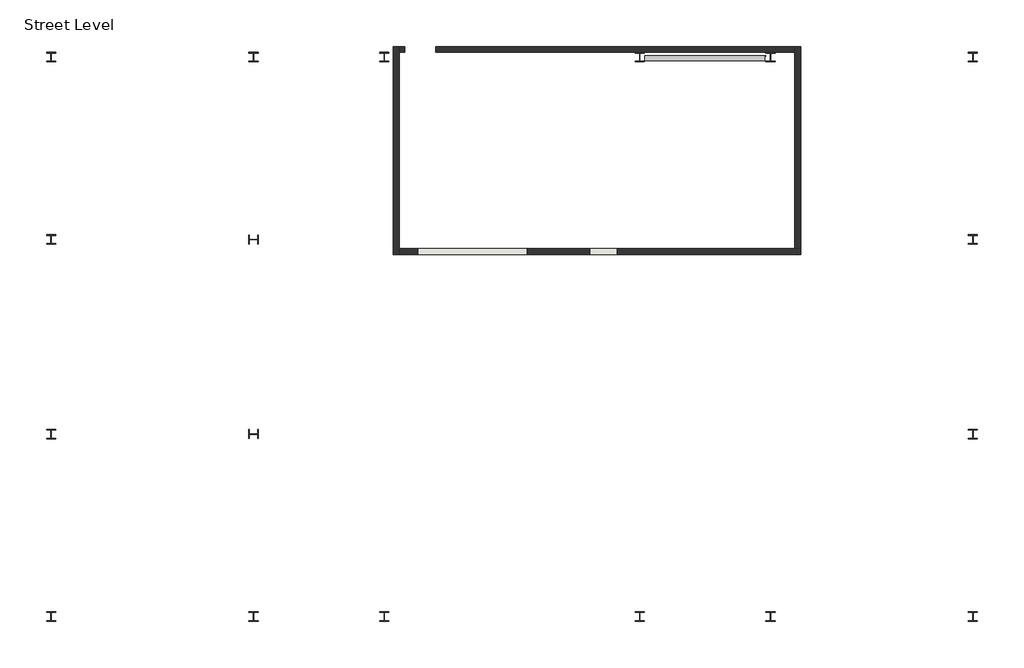
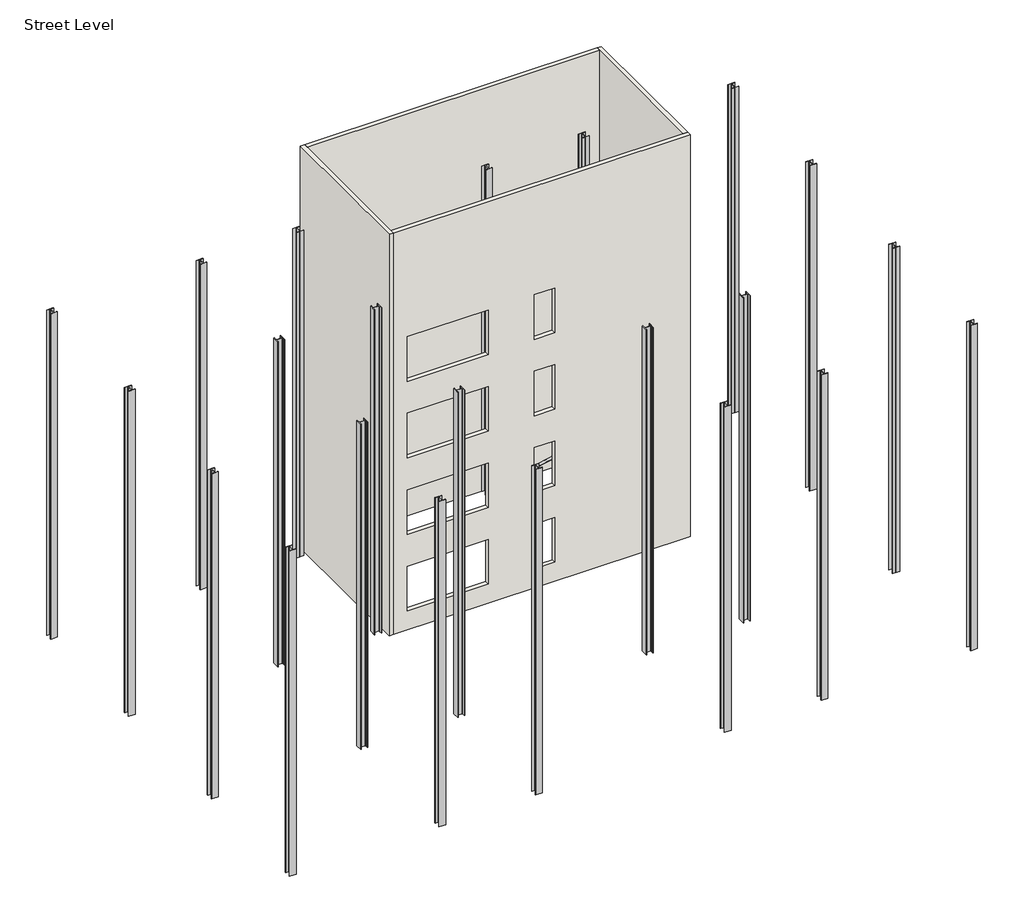
# One storey: 24 columns, 4 walls, 1 member.
"""IFC4 building model written with IfcOpenShell, lengths in millimetres."""

import ifcopenshell
import ifcopenshell.guid

model = None  # the IFC model being written
_history = None  # IfcOwnerHistory: only IFC2X3 demands one
_inside = {}  # id of a spatial element -> (the spatial element, [elements in it])
_under = {}  # id of a project, library or spatial element -> (it, [spatial elements below it])
_declared = {}  # id of a project -> (the project, [libraries it declares])
_typed = {}  # id of a type object -> (the type object, [elements of that type])
_made_of = {}  # id of a material, layer set ... -> (it, [elements and type objects made of it])


def new_model(schema):
    """Start an empty IFC model of exactly this schema.

    Asked for "IFC4X3", IfcOpenShell would pick the latest addendum, in which some entities
    have other attributes; the version numbers below select the first issue.
    IFC2X3 requires an IfcOwnerHistory on every rooted entity: one is made here for all.
    """
    global model, _history
    if schema == "IFC4X3":
        model = ifcopenshell.file(schema_version=(4, 3, 0, 0))
    else:
        model = ifcopenshell.file(schema=schema)
    _inside.clear()
    _under.clear()
    _declared.clear()
    _typed.clear()
    _made_of.clear()
    _history = None
    if model.schema == "IFC2X3":
        org = make("IfcOrganization", Name="unknown")
        user = make(
            "IfcPersonAndOrganization",
            ThePerson=make("IfcPerson", FamilyName="unknown"),
            TheOrganization=org,
        )
        app = make(
            "IfcApplication",
            ApplicationDeveloper=org,
            Version="unknown",
            ApplicationFullName="unknown",
            ApplicationIdentifier="unknown",
        )
        _history = make(
            "IfcOwnerHistory",
            OwningUser=user,
            OwningApplication=app,
            ChangeAction="ADDED",
            CreationDate=0,
        )
    return model


def make(cls, **values):
    """One entity of the class cls with the attributes given. An attribute that is None is left unset."""
    return model.create_entity(
        cls, **{name: value for name, value in values.items() if value is not None}
    )


def rooted(cls, **values):
    """An entity with a GlobalId (a new one), such as an element, a storey or a relation."""
    return make(cls, GlobalId=ifcopenshell.guid.new(), OwnerHistory=_history, **values)


def si_unit(unit_type, name, prefix=None):
    """IfcSIUnit, for example si_unit("LENGTHUNIT", "METRE", prefix="MILLI")."""
    return make("IfcSIUnit", UnitType=unit_type, Prefix=prefix, Name=name)


def assignment(units):
    """IfcUnitAssignment: the units of a project."""
    return None if units is None else make("IfcUnitAssignment", Units=units)


def point(xyz):
    """IfcCartesianPoint."""
    return None if xyz is None else make("IfcCartesianPoint", Coordinates=xyz)


def direction(xyz):
    """IfcDirection."""
    return None if xyz is None else make("IfcDirection", DirectionRatios=xyz)


def frame(location, z_axis=None, x_axis=None):
    """IfcAxis2Placement3D, a coordinate frame: its origin and axes. An axis left out is left unset."""
    return make(
        "IfcAxis2Placement3D",
        Location=point(location),
        Axis=direction(z_axis),
        RefDirection=direction(x_axis),
    )


def frame_2d(location, x_axis=None):
    """IfcAxis2Placement2D, a coordinate frame in the plane: its origin and x axis."""
    return make(
        "IfcAxis2Placement2D", Location=point(location), RefDirection=direction(x_axis)
    )


def origin():
    """The frame at (0, 0, 0) with its axes left unset."""
    return frame((0.0, 0.0, 0.0))


def place(relative_to, where):
    """IfcLocalPlacement: puts the frame where relative to a parent placement (None: the world)."""
    return make(
        "IfcLocalPlacement", PlacementRelTo=relative_to, RelativePlacement=where
    )


def context(
    kind, dimensions, precision=None, world=None, true_north=None, identifier=None
):
    """IfcGeometricRepresentationContext, for example the 3D "Model" context."""
    return make(
        "IfcGeometricRepresentationContext",
        ContextIdentifier=identifier,
        ContextType=kind,
        CoordinateSpaceDimension=dimensions,
        Precision=precision,
        WorldCoordinateSystem=world,
        TrueNorth=true_north,
    )


def project(units=None, contexts=None):
    """IfcProject with its units and contexts."""
    return rooted(
        "IfcProject",
        Name="project",
        RepresentationContexts=contexts,
        UnitsInContext=assignment(units),
    )


def spatial(cls, under=None, at=None, **own):
    """A site, building, storey or space (cls), placed at a placement, below another one or the project."""
    s = rooted(cls, ObjectPlacement=at, **own)
    if under is not None:
        _under.setdefault(under.id(), (under, []))[1].append(s)
    return s


def polyline(points):
    """IfcPolyline through the points."""
    return make("IfcPolyline", Points=[point(p) for p in points])


def circle_curve(where, radius):
    """IfcCircle in the frame where."""
    return make("IfcCircle", Position=where, Radius=radius)


def trimmed(basis, trim1, trim2, sense, master):
    """IfcTrimmedCurve: the piece of a basis curve between two trims."""
    return make(
        "IfcTrimmedCurve",
        BasisCurve=basis,
        Trim1=trim1,
        Trim2=trim2,
        SenseAgreement=sense,
        MasterRepresentation=master,
    )


def segment(curve, same_sense, transition):
    """IfcCompositeCurveSegment."""
    return make(
        "IfcCompositeCurveSegment",
        Transition=transition,
        SameSense=same_sense,
        ParentCurve=curve,
    )


def composite_curve(segments, self_intersect=None):
    """IfcCompositeCurve: segments joined end to end."""
    return make("IfcCompositeCurve", Segments=segments, SelfIntersect=self_intersect)


def outline(outer, holes=None, kind="AREA"):
    """IfcArbitraryClosedProfileDef: a profile drawn as a closed curve; with holes, ...WithVoids."""
    if holes is None:
        return make("IfcArbitraryClosedProfileDef", ProfileType=kind, OuterCurve=outer)
    return make(
        "IfcArbitraryProfileDefWithVoids",
        ProfileType=kind,
        OuterCurve=outer,
        InnerCurves=holes,
    )


def extrude(swept, where, along, depth):
    """IfcExtrudedAreaSolid: the profile swept, set in the frame where, extruded along a direction by depth."""
    return make(
        "IfcExtrudedAreaSolid",
        SweptArea=swept,
        Position=where,
        ExtrudedDirection=direction(along),
        Depth=depth,
    )


def faces_of(points, faces, orient=None, outer=None):
    """IfcFace entities. A face is a list of loops; a loop is a list of indices into points, from 0.

    orient and outer hold one flag for each loop. By default every Orientation is true, the
    first loop of a face is its IfcFaceOuterBound and the others are IfcFaceBound.
    """
    made = []
    for i, loops in enumerate(faces):
        bounds = []
        for j, loop in enumerate(loops):
            is_outer = j == 0 if outer is None else outer[i][j]
            bounds.append(
                make(
                    "IfcFaceOuterBound" if is_outer else "IfcFaceBound",
                    Bound=make("IfcPolyLoop", Polygon=[points[k] for k in loop]),
                    Orientation=True if orient is None else orient[i][j],
                )
            )
        made.append(make("IfcFace", Bounds=bounds))
    return made


def faceted_brep(points, faces, orient=None, outer=None, voids=None):
    """IfcFacetedBrep: a solid bounded by flat faces; with voids (closed shells), ...WithVoids."""
    shared = [point(p) for p in points]
    hull = make("IfcClosedShell", CfsFaces=faces_of(shared, faces, orient, outer))
    if voids is None:
        return make("IfcFacetedBrep", Outer=hull)
    return make(
        "IfcFacetedBrepWithVoids",
        Outer=hull,
        Voids=[
            make(cls, CfsFaces=faces_of(shared, fs, o, b)) for cls, fs, o, b in voids
        ],
    )


def shape(context_of_items, identifier, shape_type, items):
    """IfcShapeRepresentation: the items that make up one representation, for example the "Body"."""
    return make(
        "IfcShapeRepresentation",
        ContextOfItems=context_of_items,
        RepresentationIdentifier=identifier,
        RepresentationType=shape_type,
        Items=items,
    )


def source(mapping_origin, context_of_items, identifier, shape_type, items):
    """IfcRepresentationMap: a shape defined once, which mapped items show again and again."""
    return make(
        "IfcRepresentationMap",
        MappingOrigin=mapping_origin,
        MappedRepresentation=shape(context_of_items, identifier, shape_type, items),
    )


def transform(
    local_origin,
    x_axis=None,
    y_axis=None,
    z_axis=None,
    scale=None,
    scale2=None,
    scale3=None,
    uniform=True,
):
    """IfcCartesianTransformationOperator3D, or its non-uniform kind. x_axis, y_axis, z_axis: its Axis1, 2, 3."""
    if uniform:
        return make(
            "IfcCartesianTransformationOperator3D",
            Axis1=direction(x_axis),
            Axis2=direction(y_axis),
            LocalOrigin=point(local_origin),
            Scale=scale,
            Axis3=direction(z_axis),
        )
    return make(
        "IfcCartesianTransformationOperator3DnonUniform",
        Axis1=direction(x_axis),
        Axis2=direction(y_axis),
        LocalOrigin=point(local_origin),
        Scale=scale,
        Axis3=direction(z_axis),
        Scale2=scale2,
        Scale3=scale3,
    )


def mapped(mapping_source, mapping_target):
    """IfcMappedItem: shows the shape of a source again, moved by a transform."""
    return make(
        "IfcMappedItem", MappingSource=mapping_source, MappingTarget=mapping_target
    )


def made_of(thing, what):
    """Note that an element or type object is made of a material, layer set ...; save() writes the relation."""
    if what is not None:
        _made_of.setdefault(what.id(), (what, []))[1].append(thing)
    return thing


def element(
    cls,
    number,
    at=None,
    inside=None,
    cuts=None,
    type_object=None,
    material=None,
    context=None,
    identifier="Body",
    shape_type=None,
    held_by="IfcProductDefinitionShape",
    body=None,
    shapes=None,
    **own,
):
    """One element of the class cls, such as IfcWall. Its Tag is "e" and its number.

    at: its placement. inside: the storey or other place that contains it. cuts: it is an
    opening in that element (IfcRelVoidsElement). A single representation is given by context,
    identifier, shape_type and body (its items); several are given by shapes. held_by: the class
    of the entity that holds the representations. save() writes the other relations.
    """
    e = rooted(cls, Tag="e%d" % number, ObjectPlacement=at, **own)
    if body is not None:
        shapes = [shape(context, identifier, shape_type, body)]
    if shapes is not None:
        e.Representation = make(held_by, Representations=shapes)
    if inside is not None:
        _inside.setdefault(inside.id(), (inside, []))[1].append(e)
    if cuts is not None:
        rooted(
            "IfcRelVoidsElement", RelatingBuildingElement=cuts, RelatedOpeningElement=e
        )
    if type_object is not None:
        _typed.setdefault(type_object.id(), (type_object, []))[1].append(e)
    return made_of(e, material)


def aggregate(whole, parts):
    """IfcRelAggregates: a whole, such as a stair, and the parts it consists of."""
    return rooted("IfcRelAggregates", RelatingObject=whole, RelatedObjects=parts)


def save(model, path):
    """Write the relations noted so far, then the file.

    IfcRelAggregates (storeys below a building ...), IfcRelContainedInSpatialStructure (elements
    in a storey), IfcRelDefinesByType, IfcRelAssociatesMaterial and IfcRelDeclares: one each for
    every whole, place, type object, material and project.
    """
    for whole, parts in _under.values():
        aggregate(whole, parts)
    for where, things in _inside.values():
        rooted(
            "IfcRelContainedInSpatialStructure",
            RelatedElements=things,
            RelatingStructure=where,
        )
    for kind, things in _typed.values():
        rooted("IfcRelDefinesByType", RelatedObjects=things, RelatingType=kind)
    for what, things in _made_of.values():
        rooted("IfcRelAssociatesMaterial", RelatedObjects=things, RelatingMaterial=what)
    for by, libraries in _declared.values():
        rooted("IfcRelDeclares", RelatingContext=by, RelatedDefinitions=libraries)
    model.write(path)


def w_wide_flange_column_w12x87_da20b1fb(model_context):
    return source(origin(), model_context, "Body", "SweptSolid", [
        extrude(outline(composite_curve([segment(polyline([(153.9875, 159.146875), (153.9875, 138.6085937), (28.8726562, 138.6085937)]), True, "CONTINUOUS"), segment(trimmed(circle_curve(frame_2d((28.8726562, 116.284375)), 22.3242188), [point((28.8726562, 138.6085937))], [point((6.5484375, 116.284375))], True, "CARTESIAN"), True, "CONTINUOUS"), segment(polyline([(6.5484375, 116.284375), (6.5484375, -116.284375)]), True, "CONTINUOUS"), segment(trimmed(circle_curve(frame_2d((28.8726562, -116.284375)), 22.3242188), [point((6.5484375, -116.284375))], [point((28.8726562, -138.6085937))], True, "CARTESIAN"), True, "CONTINUOUS"), segment(polyline([(28.8726562, -138.6085937), (153.9875, -138.6085937), (153.9875, -159.146875), (-153.9875, -159.146875), (-153.9875, -138.6085937), (-28.8726563, -138.6085937)]), True, "CONTINUOUS"), segment(trimmed(circle_curve(frame_2d((-28.8726563, -116.284375)), 22.3242188), [point((-28.8726563, -138.6085937))], [point((-6.5484375, -116.284375))], True, "CARTESIAN"), True, "CONTINUOUS"), segment(polyline([(-6.5484375, -116.284375), (-6.5484375, 116.284375)]), True, "CONTINUOUS"), segment(trimmed(circle_curve(frame_2d((-28.8726563, 116.284375)), 22.3242188), [point((-6.5484375, 116.284375))], [point((-28.8726563, 138.6085937))], True, "CARTESIAN"), True, "CONTINUOUS"), segment(polyline([(-28.8726563, 138.6085937), (-153.9875, 138.6085937), (-153.9875, 159.146875), (153.9875, 159.146875)]), True, "CONTINUOUS")], self_intersect=False)), frame((0.0, 0.0, -914.4), z_axis=(0.0, 0.0, 1.0), x_axis=(1.0, 0.0, 0.0)), (0.0, 0.0, 1.0), 15544.8),
    ])


def l_angle2_l6x6x3_8_670392f0(model_context):
    return source(origin(), model_context, "Body", "SweptSolid", [
        extrude(outline(composite_curve([segment(polyline([(41.148, 41.148), (41.148, -111.252)]), True, "CONTINUOUS"), segment(trimmed(circle_curve(frame_2d((41.148, -101.727)), 9.525), [point((41.148, -111.252))], [point((31.623, -101.727))], False, "CARTESIAN"), True, "CONTINUOUS"), segment(polyline([(31.623, -101.727), (31.623, 22.098)]), True, "CONTINUOUS"), segment(trimmed(circle_curve(frame_2d((22.098, 22.098)), 9.525), [point((31.623, 22.098))], [point((22.098, 31.623))], True, "CARTESIAN"), True, "CONTINUOUS"), segment(polyline([(22.098, 31.623), (-101.727, 31.623)]), True, "CONTINUOUS"), segment(trimmed(circle_curve(frame_2d((-101.727, 41.148)), 9.525), [point((-101.727, 31.623))], [point((-111.252, 41.148))], False, "CARTESIAN"), True, "CONTINUOUS"), segment(polyline([(-111.252, 41.148), (41.148, 41.148)]), True, "CONTINUOUS")], self_intersect=False)), frame((-2053.0970548, 0.0, 0.0), z_axis=(1.0, 0.0, 0.0), x_axis=(0.0, 1.0, 0.0)), (0.0, 0.0, 1.0), 4091.5211794),
    ])


model = new_model("IFC4")

# Units and contexts
model_context = context("Model", 3, world=origin())
ifc_project = project(units=[si_unit("LENGTHUNIT", "METRE", prefix="MILLI")], contexts=[model_context])

# Site, building, storey
site = spatial("IfcSite", under=ifc_project)
building = spatial("IfcBuilding", under=site)
storey = spatial("IfcBuildingStorey", under=building, Name="Street Level", Elevation=-914.4)

# Columns
placement = place(None, origin())
w_wide_flange_column_w12x87_shape = w_wide_flange_column_w12x87_da20b1fb(model_context)
element("IfcColumn", 1, ObjectType="W-Wide Flange-Column : W12X87", at=placement, inside=storey, context=model_context, shape_type="MappedRepresentation", body=[
    mapped(w_wide_flange_column_w12x87_shape, transform((-9801.8122732, -3408.4984696, 0.0), x_axis=(0.0, -1.0, 0.0), y_axis=(1.0, 0.0, 0.0), z_axis=(0.0, 0.0, 1.0))),
])
element("IfcColumn", 2, ObjectType="W-Wide Flange-Column : W12X87", at=placement, inside=storey, context=model_context, shape_type="MappedRepresentation", body=[
    mapped(w_wide_flange_column_w12x87_shape, transform((-5433.0122732, -3408.4984696, 0.0), x_axis=(0.0, -1.0, 0.0), y_axis=(1.0, 0.0, 0.0), z_axis=(0.0, 0.0, 1.0))),
])
element("IfcColumn", 3, ObjectType="W-Wide Flange-Column : W12X87", at=placement, inside=storey, context=model_context, shape_type="MappedRepresentation", body=[
    mapped(w_wide_flange_column_w12x87_shape, transform((3101.3877268, -3408.4984696, 0.0), x_axis=(0.0, -1.0, 0.0), y_axis=(1.0, 0.0, 0.0), z_axis=(0.0, 0.0, 1.0))),
])
element("IfcColumn", 4, ObjectType="W-Wide Flange-Column : W12X87", at=placement, inside=storey, context=model_context, shape_type="MappedRepresentation", body=[
    mapped(w_wide_flange_column_w12x87_shape, transform((7470.1877268, -3408.4984696, 0.0), x_axis=(0.0, -1.0, 0.0), y_axis=(1.0, 0.0, 0.0), z_axis=(0.0, 0.0, 1.0))),
])
element("IfcColumn", 5, ObjectType="W-Wide Flange-Column : W12X87", at=placement, inside=storey, context=model_context, shape_type="MappedRepresentation", body=[
    mapped(w_wide_flange_column_w12x87_shape, transform((-9801.8122732, 3093.9015304, 0.0), x_axis=(0.0, -1.0, 0.0), y_axis=(1.0, 0.0, 0.0), z_axis=(0.0, 0.0, 1.0))),
])
element("IfcColumn", 6, ObjectType="W-Wide Flange-Column : W12X87", at=placement, inside=storey, context=model_context, shape_type="MappedRepresentation", body=[
    mapped(w_wide_flange_column_w12x87_shape, transform((-5433.0122732, 3093.9015304, 0.0), x_axis=(0.0, -1.0, 0.0), y_axis=(1.0, 0.0, 0.0), z_axis=(0.0, 0.0, 1.0))),
])
element("IfcColumn", 7, ObjectType="W-Wide Flange-Column : W12X87", at=placement, inside=storey, context=model_context, shape_type="MappedRepresentation", body=[
    mapped(w_wide_flange_column_w12x87_shape, transform((3101.3877268, 3093.9015304, 0.0), x_axis=(0.0, -1.0, 0.0), y_axis=(1.0, 0.0, 0.0), z_axis=(0.0, 0.0, 1.0))),
])
element("IfcColumn", 8, ObjectType="W-Wide Flange-Column : W12X87", at=placement, inside=storey, context=model_context, shape_type="MappedRepresentation", body=[
    mapped(w_wide_flange_column_w12x87_shape, transform((7470.1877268, 3093.9015304, 0.0), x_axis=(0.0, -1.0, 0.0), y_axis=(1.0, 0.0, 0.0), z_axis=(0.0, 0.0, 1.0))),
])
element("IfcColumn", 9, ObjectType="W-Wide Flange-Column : W12X87", at=placement, inside=storey, context=model_context, shape_type="MappedRepresentation", body=[
    mapped(w_wide_flange_column_w12x87_shape, transform((-16558.2122732, 9189.9015304, 0.0), x_axis=(1.0, 0.0, 0.0), y_axis=(0.0, 1.0, 0.0), z_axis=(0.0, 0.0, 1.0))),
])
element("IfcColumn", 10, ObjectType="W-Wide Flange-Column : W12X87", at=placement, inside=storey, context=model_context, shape_type="MappedRepresentation", body=[
    mapped(w_wide_flange_column_w12x87_shape, transform((-16558.2122732, 3093.9015304, 0.0), x_axis=(1.0, 0.0, 0.0), y_axis=(0.0, 1.0, 0.0), z_axis=(0.0, 0.0, 1.0))),
])
element("IfcColumn", 11, ObjectType="W-Wide Flange-Column : W12X87", at=placement, inside=storey, context=model_context, shape_type="MappedRepresentation", body=[
    mapped(w_wide_flange_column_w12x87_shape, transform((-9801.8122732, 9189.9015304, 0.0), x_axis=(1.0, 0.0, 0.0), y_axis=(0.0, 1.0, 0.0), z_axis=(0.0, 0.0, 1.0))),
])
element("IfcColumn", 12, ObjectType="W-Wide Flange-Column : W12X87", at=placement, inside=storey, context=model_context, shape_type="MappedRepresentation", body=[
    mapped(w_wide_flange_column_w12x87_shape, transform((-5433.0122732, 9189.9015304, 0.0), x_axis=(1.0, 0.0, 0.0), y_axis=(0.0, 1.0, 0.0), z_axis=(0.0, 0.0, 1.0))),
])
element("IfcColumn", 13, ObjectType="W-Wide Flange-Column : W12X87", at=placement, inside=storey, context=model_context, shape_type="MappedRepresentation", body=[
    mapped(w_wide_flange_column_w12x87_shape, transform((3101.3877268, 9189.9015304, 0.0), x_axis=(1.0, 0.0, 0.0), y_axis=(0.0, 1.0, 0.0), z_axis=(0.0, 0.0, 1.0))),
])
element("IfcColumn", 14, ObjectType="W-Wide Flange-Column : W12X87", at=placement, inside=storey, context=model_context, shape_type="MappedRepresentation", body=[
    mapped(w_wide_flange_column_w12x87_shape, transform((7470.1877268, 9189.9015304, 0.0), x_axis=(1.0, 0.0, 0.0), y_axis=(0.0, 1.0, 0.0), z_axis=(0.0, 0.0, 1.0))),
])
element("IfcColumn", 15, ObjectType="W-Wide Flange-Column : W12X87", at=placement, inside=storey, context=model_context, shape_type="MappedRepresentation", body=[
    mapped(w_wide_flange_column_w12x87_shape, transform((14226.5877268, 9189.9015304, 0.0), x_axis=(1.0, 0.0, 0.0), y_axis=(0.0, 1.0, 0.0), z_axis=(0.0, 0.0, 1.0))),
])
element("IfcColumn", 16, ObjectType="W-Wide Flange-Column : W12X87", at=placement, inside=storey, context=model_context, shape_type="MappedRepresentation", body=[
    mapped(w_wide_flange_column_w12x87_shape, transform((14226.5877268, 3093.9015304, 0.0), x_axis=(1.0, 0.0, 0.0), y_axis=(0.0, 1.0, 0.0), z_axis=(0.0, 0.0, 1.0))),
])
element("IfcColumn", 17, ObjectType="W-Wide Flange-Column : W12X87", at=placement, inside=storey, context=model_context, shape_type="MappedRepresentation", body=[
    mapped(w_wide_flange_column_w12x87_shape, transform((14226.5877268, -3408.4984696, 0.0), x_axis=(1.0, 0.0, 0.0), y_axis=(0.0, 1.0, 0.0), z_axis=(0.0, 0.0, 1.0))),
])
element("IfcColumn", 18, ObjectType="W-Wide Flange-Column : W12X87", at=placement, inside=storey, context=model_context, shape_type="MappedRepresentation", body=[
    mapped(w_wide_flange_column_w12x87_shape, transform((14226.5877268, -9504.4984696, 0.0), x_axis=(1.0, 0.0, 0.0), y_axis=(0.0, 1.0, 0.0), z_axis=(0.0, 0.0, 1.0))),
])
element("IfcColumn", 19, ObjectType="W-Wide Flange-Column : W12X87", at=placement, inside=storey, context=model_context, shape_type="MappedRepresentation", body=[
    mapped(w_wide_flange_column_w12x87_shape, transform((7470.1877268, -9504.4984696, 0.0), x_axis=(1.0, 0.0, 0.0), y_axis=(0.0, 1.0, 0.0), z_axis=(0.0, 0.0, 1.0))),
])
element("IfcColumn", 20, ObjectType="W-Wide Flange-Column : W12X87", at=placement, inside=storey, context=model_context, shape_type="MappedRepresentation", body=[
    mapped(w_wide_flange_column_w12x87_shape, transform((3101.3877268, -9504.4984696, 0.0), x_axis=(1.0, 0.0, 0.0), y_axis=(0.0, 1.0, 0.0), z_axis=(0.0, 0.0, 1.0))),
])
element("IfcColumn", 21, ObjectType="W-Wide Flange-Column : W12X87", at=placement, inside=storey, context=model_context, shape_type="MappedRepresentation", body=[
    mapped(w_wide_flange_column_w12x87_shape, transform((-5433.0122732, -9504.4984696, 0.0), x_axis=(1.0, 0.0, 0.0), y_axis=(0.0, 1.0, 0.0), z_axis=(0.0, 0.0, 1.0))),
])
element("IfcColumn", 22, ObjectType="W-Wide Flange-Column : W12X87", at=placement, inside=storey, context=model_context, shape_type="MappedRepresentation", body=[
    mapped(w_wide_flange_column_w12x87_shape, transform((-9801.8122732, -9504.4984696, 0.0), x_axis=(1.0, 0.0, 0.0), y_axis=(0.0, 1.0, 0.0), z_axis=(0.0, 0.0, 1.0))),
])
element("IfcColumn", 23, ObjectType="W-Wide Flange-Column : W12X87", at=placement, inside=storey, context=model_context, shape_type="MappedRepresentation", body=[
    mapped(w_wide_flange_column_w12x87_shape, transform((-16558.2122732, -9504.4984696, 0.0), x_axis=(1.0, 0.0, 0.0), y_axis=(0.0, 1.0, 0.0), z_axis=(0.0, 0.0, 1.0))),
])
element("IfcColumn", 24, ObjectType="W-Wide Flange-Column : W12X87", at=placement, inside=storey, context=model_context, shape_type="MappedRepresentation", body=[
    mapped(w_wide_flange_column_w12x87_shape, transform((-16558.2122732, -3408.4984696, 0.0), x_axis=(1.0, 0.0, 0.0), y_axis=(0.0, 1.0, 0.0), z_axis=(0.0, 0.0, 1.0))),
])

# Member
l_angle2_l6x6x3_8_shape = l_angle2_l6x6x3_8_670392f0(model_context)
element("IfcMember", 25, ObjectType="L-Angle2 : L6X6X3/8", at=placement, inside=storey, context=model_context, shape_type="MappedRepresentation", body=[
    mapped(l_angle2_l6x6x3_8_shape, transform((5285.7877268, 9189.9015304, -457.2), x_axis=(0.9787906252528689, 0.0, 0.20486315412269337), y_axis=(0.0, 1.0000000000000002, 0.0), z_axis=(-0.20486315412269337, 0.0, 0.9787906252528689))),
])

# Walls
element("IfcWall", 26, ObjectType="Generic - 8\" Masonry", at=placement, inside=storey, context=model_context, shape_type="Brep", body=[
    faceted_brep([(-5128.2122732, 9545.5015304, -914.4), (-5128.2122732, 2595.4265304, -914.4), (-5128.2122732, 2595.4265304, 18288.0), (-5128.2122732, 9545.5015304, 18288.0), (-4934.5372732, 9545.5015304, -914.4), (-4934.5372732, 9545.5015304, 18288.0), (-4934.5372732, 9351.8265304, 18288.0), (-4934.5372732, 2789.1015304, 18288.0), (-4934.5372732, 2595.4265304, 18288.0), (-4934.5372732, 2595.4265304, -914.4), (-4934.5372732, 2789.1015304, -914.4), (-4934.5372732, 9351.8265304, -914.4)], [[[0, 1, 2, 3]], [[4, 5, 6, 7, 8, 9, 10, 11]], [[1, 0, 4, 11, 10, 9]], [[3, 2, 8, 7, 6, 5]], [[0, 3, 5, 4]], [[2, 1, 9, 8]]]),
])
element("IfcWall", 27, ObjectType="Generic - 8\" Masonry", at=placement, inside=storey, context=model_context, shape_type="Brep", body=[
    faceted_brep([(8476.6627268, 2789.1015304, -914.4), (8282.9877268, 2789.1015304, -914.4), (-4934.5372732, 2789.1015304, -914.4), (-4934.5372732, 2789.1015304, 18288.0), (8282.9877268, 2789.1015304, 18288.0), (8476.6627268, 2789.1015304, 18288.0), (-653.0497732, 2789.1015304, 2133.6), (-4310.6497732, 2789.1015304, 2133.6), (-4310.6497732, 2789.1015304, 0.0), (-653.0497732, 2789.1015304, 0.0), (2344.1502268, 2789.1015304, 2133.6), (1429.7502268, 2789.1015304, 2133.6), (1429.7502268, 2789.1015304, 0.0), (2344.1502268, 2789.1015304, 0.0), (-653.0497732, 2789.1015304, 5791.2), (-4310.6497732, 2789.1015304, 5791.2), (-4310.6497732, 2789.1015304, 3657.6), (-653.0497732, 2789.1015304, 3657.6), (2344.1502268, 2789.1015304, 5791.2), (1429.7502268, 2789.1015304, 5791.2), (1429.7502268, 2789.1015304, 3657.6), (2344.1502268, 2789.1015304, 3657.6), (-653.0497732, 2789.1015304, 9448.8), (-4310.6497732, 2789.1015304, 9448.8), (-4310.6497732, 2789.1015304, 7315.2), (-653.0497732, 2789.1015304, 7315.2), (2344.1502268, 2789.1015304, 9448.8), (1429.7502268, 2789.1015304, 9448.8), (1429.7502268, 2789.1015304, 7315.2), (2344.1502268, 2789.1015304, 7315.2), (-653.0497732, 2789.1015304, 13106.4), (-4310.6497732, 2789.1015304, 13106.4), (-4310.6497732, 2789.1015304, 10972.8), (-653.0497732, 2789.1015304, 10972.8), (2344.1502268, 2789.1015304, 13106.4), (1429.7502268, 2789.1015304, 13106.4), (1429.7502268, 2789.1015304, 10972.8), (2344.1502268, 2789.1015304, 10972.8), (-4934.5372732, 2595.4265304, -914.4), (8476.6627268, 2595.4265304, -914.4), (8476.6627268, 2595.4265304, 18288.0), (-4934.5372732, 2595.4265304, 18288.0), (-4310.6497732, 2595.4265304, 2133.6), (-653.0497732, 2595.4265304, 2133.6), (-653.0497732, 2595.4265304, 0.0), (-4310.6497732, 2595.4265304, 0.0), (1429.7502268, 2595.4265304, 2133.6), (2344.1502268, 2595.4265304, 2133.6), (2344.1502268, 2595.4265304, 0.0), (1429.7502268, 2595.4265304, 0.0), (-4310.6497732, 2595.4265304, 5791.2), (-653.0497732, 2595.4265304, 5791.2), (-653.0497732, 2595.4265304, 3657.6), (-4310.6497732, 2595.4265304, 3657.6), (1429.7502268, 2595.4265304, 5791.2), (2344.1502268, 2595.4265304, 5791.2), (2344.1502268, 2595.4265304, 3657.6), (1429.7502268, 2595.4265304, 3657.6), (-4310.6497732, 2595.4265304, 9448.8), (-653.0497732, 2595.4265304, 9448.8), (-653.0497732, 2595.4265304, 7315.2), (-4310.6497732, 2595.4265304, 7315.2), (1429.7502268, 2595.4265304, 9448.8), (2344.1502268, 2595.4265304, 9448.8), (2344.1502268, 2595.4265304, 7315.2), (1429.7502268, 2595.4265304, 7315.2), (-4310.6497732, 2595.4265304, 13106.4), (-653.0497732, 2595.4265304, 13106.4), (-653.0497732, 2595.4265304, 10972.8), (-4310.6497732, 2595.4265304, 10972.8), (1429.7502268, 2595.4265304, 13106.4), (2344.1502268, 2595.4265304, 13106.4), (2344.1502268, 2595.4265304, 10972.8), (1429.7502268, 2595.4265304, 10972.8)], [[[0, 1, 2, 3, 4, 5], [6, 7, 8, 9], [10, 11, 12, 13], [14, 15, 16, 17], [18, 19, 20, 21], [22, 23, 24, 25], [26, 27, 28, 29], [30, 31, 32, 33], [34, 35, 36, 37]], [[38, 39, 40, 41], [42, 43, 44, 45], [46, 47, 48, 49], [50, 51, 52, 53], [54, 55, 56, 57], [58, 59, 60, 61], [62, 63, 64, 65], [66, 67, 68, 69], [70, 71, 72, 73]], [[2, 1, 0, 39, 38]], [[5, 4, 3, 41, 40]], [[0, 5, 40, 39]], [[3, 2, 38, 41]], [[6, 43, 42, 7]], [[8, 45, 44, 9]], [[43, 6, 9, 44]], [[7, 42, 45, 8]], [[10, 47, 46, 11]], [[12, 49, 48, 13]], [[47, 10, 13, 48]], [[11, 46, 49, 12]], [[14, 51, 50, 15]], [[16, 53, 52, 17]], [[51, 14, 17, 52]], [[15, 50, 53, 16]], [[18, 55, 54, 19]], [[20, 57, 56, 21]], [[55, 18, 21, 56]], [[19, 54, 57, 20]], [[22, 59, 58, 23]], [[24, 61, 60, 25]], [[59, 22, 25, 60]], [[23, 58, 61, 24]], [[26, 63, 62, 27]], [[28, 65, 64, 29]], [[63, 26, 29, 64]], [[27, 62, 65, 28]], [[30, 67, 66, 31]], [[32, 69, 68, 33]], [[67, 30, 33, 68]], [[31, 66, 69, 32]], [[34, 71, 70, 35]], [[36, 73, 72, 37]], [[71, 34, 37, 72]], [[35, 70, 73, 36]]]),
])
element("IfcWall", 28, ObjectType="Generic - 8\" Masonry", at=placement, inside=storey, context=model_context, shape_type="Brep", body=[
    faceted_brep([(8282.9877268, 9545.5015304, -914.4), (8282.9877268, 9351.8265304, -914.4), (8282.9877268, 2789.1015304, -914.4), (8282.9877268, 2789.1015304, 18288.0), (8282.9877268, 9351.8265304, 18288.0), (8282.9877268, 9545.5015304, 18288.0), (8476.6627268, 9545.5015304, -914.4), (8476.6627268, 9545.5015304, 18288.0), (8476.6627268, 2789.1015304, 18288.0), (8476.6627268, 2789.1015304, -914.4)], [[[0, 1, 2, 3, 4, 5]], [[6, 7, 8, 9]], [[2, 1, 0, 6, 9]], [[5, 4, 3, 8, 7]], [[0, 5, 7, 6]], [[3, 2, 9, 8]]]),
])
element("IfcWall", 29, ObjectType="Generic - 8\" Masonry", at=placement, inside=storey, context=model_context, shape_type="SweptSolid", body=[
    extrude(outline(polyline([(-914.4, 8282.9877268), (18288.0, 8282.9877268), (18288.0, -4934.5372732), (-914.4, -4934.5372732), (-914.4, -4750.3872732), (1320.8, -4750.3872732), (1320.8, -3715.3372732), (-914.4, -3715.3372732), (-914.4, 8282.9877268)])), frame((0.0, 9351.8265304, 0.0), z_axis=(0.0, 1.0, 0.0), x_axis=(0.0, 0.0, 1.0)), (0.0, 0.0, 1.0), 193.675),
])

save(model, "model.ifc")

# Revit data of these elements
# Project information
#   Organization Name = "G3B Press"
#   Organization Description = "Paul F. Aubin Cosulting Services, Inc."
#   Building Name = "Revit Essentials for Architecture"
#   Author = "Paul F. Aubin"
#   Author Website = "https://www.paulaubin.com"
#   Copyright = "Copyright © 2020 Paul F Aubin, all rights reserved"
#   Project Issue Date = "8/1/2020"
#   Project Status = "Design Development"
#   Client Name = "Links Folder Version 2"
#   Project Address = "123 State ST\nSuite 301\nChicago, IL 60606"
#   Project Name = "Commercial-Structure_V2"
#   Project Number = "2020.04S"
# Grids (mm)
#   "1.1": line (-22547.601, -8894.898) -> (19277.595, -8894.898)
#   "1": line (-22547.601, -9504.498) -> (19277.595, -9504.498)
#   "2": line (-22547.601, -3408.498) -> (19277.595, -3408.498)
#   "3": line (-22547.601, 3093.902) -> (19277.595, 3093.902)
#   "4": line (-22547.601, 9189.902) -> (19277.595, 9189.902)
#   "A": line (-16558.212, 12259.726) -> (-16558.212, -14197.104)
#   "B": line (-9801.812, 12259.726) -> (-9801.812, -14197.104)
#   "C": line (-5433.012, 12259.726) -> (-5433.012, -14197.104)
#   "D": line (3101.388, 12259.726) -> (3101.388, -14197.104)
#   "E": line (7470.188, 12259.726) -> (7470.188, -14197.104)
#   "F": line (14226.588, 12259.726) -> (14226.588, -14197.104)
#   "C.3": line (-2689.812, -15151.11) -> (-2689.812, -5965.346)
#   "C.7": line (358.188, -15151.11) -> (358.188, -5965.346)
# Type "W-Wide Flange-Column : W12X87"
#   Assembly Code = "B10"
#   A = 0.18 SF
#   W = 87
#   bf = 1' - 0 1/8"
#   d = 1' - 0 17/32"
#   k = 0' - 1 11/16"
#   kr = 0' - 0 225/256"
#   tf = 0' - 0 207/256"
#   tw = 0' - 0 33/64"
#   Structural Material [instance default] = Metal - Steel - ASTM A992
# Type "L-Angle2 : L6X6X3/8"
#   Assembly Code = "B10"
#   k = 0' - 0 7/8"
#   W = 14.9
#   Length [instance default] = 5' - 0"
#   b = 0' - 6"
#   d = 0' - 6"
#   t = 0' - 0 3/8"
#   x = 0' - 1.62"
#   y = 0' - 1.62"
#   A = 0.0304167 SF
#   Structural Material [instance default] = Steel ASTM A36
# Type "Generic - 8\" Masonry"
#   Assembly Code = "B2010"
#   Layers, outside or top first: 0' - 7 5/8" "Masonry - Concrete Masonry Units" (function 1)
# Elements 1, 2, 3, 4, 5, 6, 7, 8, 9, 10, 11, 12, 13, 14, 15, 16, 17, 18, 19, 20, 21, 22, 23, 24 (IfcColumn, "W-Wide Flange-Column : W12X87")
#   Structural Material = Metal - Steel - ASTM A992
#   Phase Created = New Construction
#   Materials on its faces: "Metal - Steel - ASTM A992"
# Element 25 (IfcMember, "L-Angle2 : L6X6X3/8")
#   Structural Material = Steel ASTM A36
#   Phase Created = New Construction
#   Materials on its faces: "Steel ASTM A36"
# Elements 26, 27, 28, 29 (IfcWall, "Generic - 8\" Masonry")
#   Top Offset = 12' - 0"
#   Base Offset = 0' - 0"
#   Unconnected Height = 63' - 0"
#   wall height = 63' - 0"
#   Phase Created = New Construction
#   Base Constraint = Street Level
#   Top Constraint = Roof
#   Materials on its faces: "Masonry - Concrete Masonry Units"
# Materials
#   "Metal - Steel - ASTM A992": class "Unassigned", colour RGB 199 199 199, transparency 0, Description = "Steel ASTM A992"
#   "Steel ASTM A36": class "Metal", colour RGB 199 199 199, transparency 0, Description = "Structural steel, ASTM A36 Grade B, mill finish", Cost = 0
#   "Masonry - Concrete Masonry Units": class "Unassigned", colour RGB 227 227 227, transparency 0, Description = "CMU"
